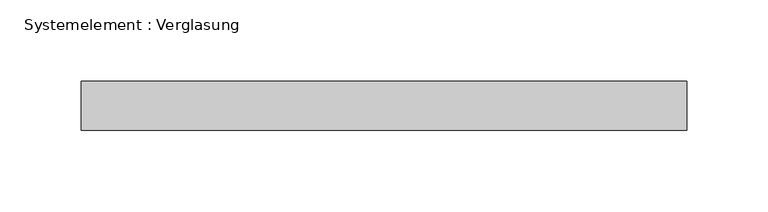
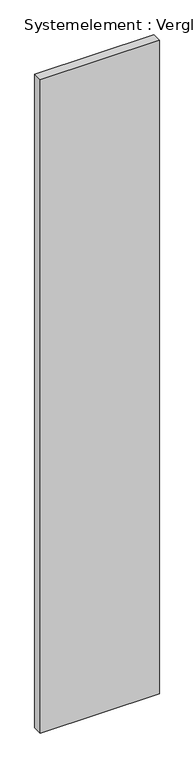
"""IFC4 building model written with IfcOpenShell, lengths in millimetres: plate geometry, Systemelement : Verglasung."""

from ifc_helpers import new_model, si_unit, origin, origin_with_axes, place, context, project, spatial, polyline, outline, extrude, source, transform, mapped, element, save


def systemelement_verglasung_a8a3d52d(model_context):
    return source(origin(), model_context, "Body", "SweptSolid", [
        extrude(outline(polyline([(186.2499998, -15.0), (-186.2499998, -15.0), (-186.2499998, 15.0), (186.2499998, 15.0), (186.2499998, -15.0)])), origin_with_axes(), (0.0, 0.0, 1.0), 2160.0),
    ])


if __name__ == "__main__":
    model = new_model("IFC4")
    model_context = context("Model", 3, world=origin())
    ifc_project = project(units=[si_unit("LENGTHUNIT", "METRE", prefix="MILLI")], contexts=[model_context])
    site = spatial("IfcSite", under=ifc_project)
    building = spatial("IfcBuilding", under=site)
    placement = place(None, origin())
    systemelement_verglasung_shape = systemelement_verglasung_a8a3d52d(model_context)
    element("IfcPlate", 1, ObjectType="Systemelement : Verglasung", at=placement, inside=building, context=model_context, shape_type="MappedRepresentation", body=[
        mapped(systemelement_verglasung_shape, transform((0.0, 0.0, 0.0), x_axis=(1.0, 0.0, 0.0), y_axis=(0.0, 1.0, 0.0), z_axis=(0.0, 0.0, 1.0))),
    ])
    save(model, "model.ifc")

# Revit data of these elements
# Type "Systemelement : Verglasung"
#   Construction Type Id = "GSP4R"
#   Analytic Construction = "1/8 Zoll Pilkington-Verglasung einfach"
#   Visual Light Transmittance = 0.9
#   Solar Heat Gain Coefficient = 0.86
#   Heat Transfer Coefficient (U) = 6.7069 W/(m²·K)
# Element 1 (IfcPlate, "Systemelement : Verglasung")
#   Materials on its faces: "Glas"
# Materials
#   "Glas": class "Glas", colour RGB 0 0 255, transparency 0.75, Comments = "Render-Darstellung nicht aktualisiert ", Cost = 0
